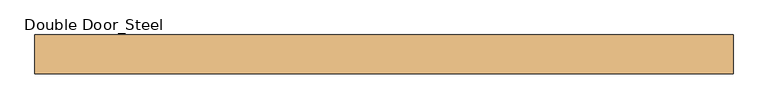
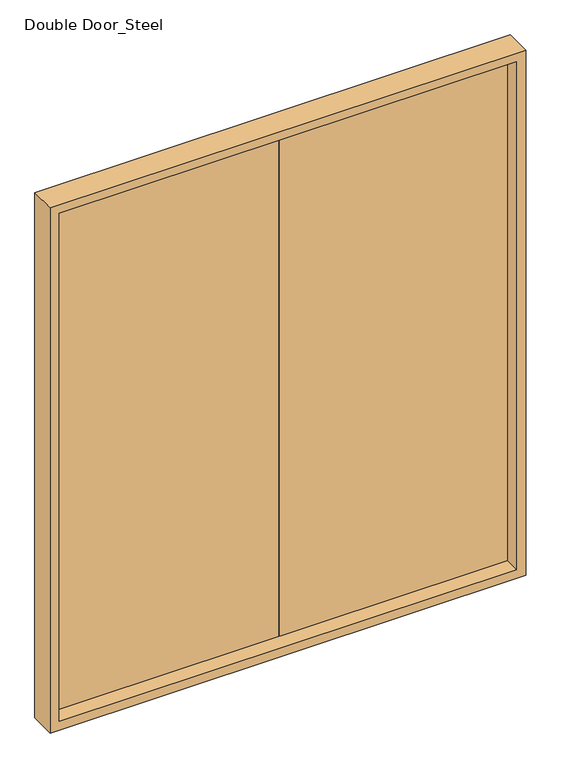
"""IFC4 building model written with IfcOpenShell, lengths in millimetres: door geometry, Double Door_Steel : H_DR_AR_B12_Double Door_Steel_W2000xH2100_0Hr."""

import ifcopenshell
import ifcopenshell.guid

model = None  # the IFC model being written
_history = None  # IfcOwnerHistory: only IFC2X3 demands one
_inside = {}  # id of a spatial element -> (the spatial element, [elements in it])
_under = {}  # id of a project, library or spatial element -> (it, [spatial elements below it])
_declared = {}  # id of a project -> (the project, [libraries it declares])
_typed = {}  # id of a type object -> (the type object, [elements of that type])
_made_of = {}  # id of a material, layer set ... -> (it, [elements and type objects made of it])


def new_model(schema):
    """Start an empty IFC model of exactly this schema.

    Asked for "IFC4X3", IfcOpenShell would pick the latest addendum, in which some entities
    have other attributes; the version numbers below select the first issue.
    IFC2X3 requires an IfcOwnerHistory on every rooted entity: one is made here for all.
    """
    global model, _history
    if schema == "IFC4X3":
        model = ifcopenshell.file(schema_version=(4, 3, 0, 0))
    else:
        model = ifcopenshell.file(schema=schema)
    _inside.clear()
    _under.clear()
    _declared.clear()
    _typed.clear()
    _made_of.clear()
    _history = None
    if model.schema == "IFC2X3":
        org = make("IfcOrganization", Name="unknown")
        user = make(
            "IfcPersonAndOrganization",
            ThePerson=make("IfcPerson", FamilyName="unknown"),
            TheOrganization=org,
        )
        app = make(
            "IfcApplication",
            ApplicationDeveloper=org,
            Version="unknown",
            ApplicationFullName="unknown",
            ApplicationIdentifier="unknown",
        )
        _history = make(
            "IfcOwnerHistory",
            OwningUser=user,
            OwningApplication=app,
            ChangeAction="ADDED",
            CreationDate=0,
        )
    return model


def make(cls, **values):
    """One entity of the class cls with the attributes given. An attribute that is None is left unset."""
    return model.create_entity(
        cls, **{name: value for name, value in values.items() if value is not None}
    )


def rooted(cls, **values):
    """An entity with a GlobalId (a new one), such as an element, a storey or a relation."""
    return make(cls, GlobalId=ifcopenshell.guid.new(), OwnerHistory=_history, **values)


def si_unit(unit_type, name, prefix=None):
    """IfcSIUnit, for example si_unit("LENGTHUNIT", "METRE", prefix="MILLI")."""
    return make("IfcSIUnit", UnitType=unit_type, Prefix=prefix, Name=name)


def assignment(units):
    """IfcUnitAssignment: the units of a project."""
    return None if units is None else make("IfcUnitAssignment", Units=units)


def point(xyz):
    """IfcCartesianPoint."""
    return None if xyz is None else make("IfcCartesianPoint", Coordinates=xyz)


def direction(xyz):
    """IfcDirection."""
    return None if xyz is None else make("IfcDirection", DirectionRatios=xyz)


def frame(location, z_axis=None, x_axis=None):
    """IfcAxis2Placement3D, a coordinate frame: its origin and axes. An axis left out is left unset."""
    return make(
        "IfcAxis2Placement3D",
        Location=point(location),
        Axis=direction(z_axis),
        RefDirection=direction(x_axis),
    )


def origin():
    """The frame at (0, 0, 0) with its axes left unset."""
    return frame((0.0, 0.0, 0.0))


def place(relative_to, where):
    """IfcLocalPlacement: puts the frame where relative to a parent placement (None: the world)."""
    return make(
        "IfcLocalPlacement", PlacementRelTo=relative_to, RelativePlacement=where
    )


def context(
    kind, dimensions, precision=None, world=None, true_north=None, identifier=None
):
    """IfcGeometricRepresentationContext, for example the 3D "Model" context."""
    return make(
        "IfcGeometricRepresentationContext",
        ContextIdentifier=identifier,
        ContextType=kind,
        CoordinateSpaceDimension=dimensions,
        Precision=precision,
        WorldCoordinateSystem=world,
        TrueNorth=true_north,
    )


def project(units=None, contexts=None):
    """IfcProject with its units and contexts."""
    return rooted(
        "IfcProject",
        Name="project",
        RepresentationContexts=contexts,
        UnitsInContext=assignment(units),
    )


def spatial(cls, under=None, at=None, **own):
    """A site, building, storey or space (cls), placed at a placement, below another one or the project."""
    s = rooted(cls, ObjectPlacement=at, **own)
    if under is not None:
        _under.setdefault(under.id(), (under, []))[1].append(s)
    return s


def polyline(points):
    """IfcPolyline through the points."""
    return make("IfcPolyline", Points=[point(p) for p in points])


def outline(outer, holes=None, kind="AREA"):
    """IfcArbitraryClosedProfileDef: a profile drawn as a closed curve; with holes, ...WithVoids."""
    if holes is None:
        return make("IfcArbitraryClosedProfileDef", ProfileType=kind, OuterCurve=outer)
    return make(
        "IfcArbitraryProfileDefWithVoids",
        ProfileType=kind,
        OuterCurve=outer,
        InnerCurves=holes,
    )


def extrude(swept, where, along, depth):
    """IfcExtrudedAreaSolid: the profile swept, set in the frame where, extruded along a direction by depth."""
    return make(
        "IfcExtrudedAreaSolid",
        SweptArea=swept,
        Position=where,
        ExtrudedDirection=direction(along),
        Depth=depth,
    )


def faces_of(points, faces, orient=None, outer=None):
    """IfcFace entities. A face is a list of loops; a loop is a list of indices into points, from 0.

    orient and outer hold one flag for each loop. By default every Orientation is true, the
    first loop of a face is its IfcFaceOuterBound and the others are IfcFaceBound.
    """
    made = []
    for i, loops in enumerate(faces):
        bounds = []
        for j, loop in enumerate(loops):
            is_outer = j == 0 if outer is None else outer[i][j]
            bounds.append(
                make(
                    "IfcFaceOuterBound" if is_outer else "IfcFaceBound",
                    Bound=make("IfcPolyLoop", Polygon=[points[k] for k in loop]),
                    Orientation=True if orient is None else orient[i][j],
                )
            )
        made.append(make("IfcFace", Bounds=bounds))
    return made


def faceted_brep(points, faces, orient=None, outer=None, voids=None):
    """IfcFacetedBrep: a solid bounded by flat faces; with voids (closed shells), ...WithVoids."""
    shared = [point(p) for p in points]
    hull = make("IfcClosedShell", CfsFaces=faces_of(shared, faces, orient, outer))
    if voids is None:
        return make("IfcFacetedBrep", Outer=hull)
    return make(
        "IfcFacetedBrepWithVoids",
        Outer=hull,
        Voids=[
            make(cls, CfsFaces=faces_of(shared, fs, o, b)) for cls, fs, o, b in voids
        ],
    )


def shape(context_of_items, identifier, shape_type, items):
    """IfcShapeRepresentation: the items that make up one representation, for example the "Body"."""
    return make(
        "IfcShapeRepresentation",
        ContextOfItems=context_of_items,
        RepresentationIdentifier=identifier,
        RepresentationType=shape_type,
        Items=items,
    )


def source(mapping_origin, context_of_items, identifier, shape_type, items):
    """IfcRepresentationMap: a shape defined once, which mapped items show again and again."""
    return make(
        "IfcRepresentationMap",
        MappingOrigin=mapping_origin,
        MappedRepresentation=shape(context_of_items, identifier, shape_type, items),
    )


def transform(
    local_origin,
    x_axis=None,
    y_axis=None,
    z_axis=None,
    scale=None,
    scale2=None,
    scale3=None,
    uniform=True,
):
    """IfcCartesianTransformationOperator3D, or its non-uniform kind. x_axis, y_axis, z_axis: its Axis1, 2, 3."""
    if uniform:
        return make(
            "IfcCartesianTransformationOperator3D",
            Axis1=direction(x_axis),
            Axis2=direction(y_axis),
            LocalOrigin=point(local_origin),
            Scale=scale,
            Axis3=direction(z_axis),
        )
    return make(
        "IfcCartesianTransformationOperator3DnonUniform",
        Axis1=direction(x_axis),
        Axis2=direction(y_axis),
        LocalOrigin=point(local_origin),
        Scale=scale,
        Axis3=direction(z_axis),
        Scale2=scale2,
        Scale3=scale3,
    )


def mapped(mapping_source, mapping_target):
    """IfcMappedItem: shows the shape of a source again, moved by a transform."""
    return make(
        "IfcMappedItem", MappingSource=mapping_source, MappingTarget=mapping_target
    )


def made_of(thing, what):
    """Note that an element or type object is made of a material, layer set ...; save() writes the relation."""
    if what is not None:
        _made_of.setdefault(what.id(), (what, []))[1].append(thing)
    return thing


def element(
    cls,
    number,
    at=None,
    inside=None,
    cuts=None,
    type_object=None,
    material=None,
    context=None,
    identifier="Body",
    shape_type=None,
    held_by="IfcProductDefinitionShape",
    body=None,
    shapes=None,
    **own,
):
    """One element of the class cls, such as IfcWall. Its Tag is "e" and its number.

    at: its placement. inside: the storey or other place that contains it. cuts: it is an
    opening in that element (IfcRelVoidsElement). A single representation is given by context,
    identifier, shape_type and body (its items); several are given by shapes. held_by: the class
    of the entity that holds the representations. save() writes the other relations.
    """
    e = rooted(cls, Tag="e%d" % number, ObjectPlacement=at, **own)
    if body is not None:
        shapes = [shape(context, identifier, shape_type, body)]
    if shapes is not None:
        e.Representation = make(held_by, Representations=shapes)
    if inside is not None:
        _inside.setdefault(inside.id(), (inside, []))[1].append(e)
    if cuts is not None:
        rooted(
            "IfcRelVoidsElement", RelatingBuildingElement=cuts, RelatedOpeningElement=e
        )
    if type_object is not None:
        _typed.setdefault(type_object.id(), (type_object, []))[1].append(e)
    return made_of(e, material)


def aggregate(whole, parts):
    """IfcRelAggregates: a whole, such as a stair, and the parts it consists of."""
    return rooted("IfcRelAggregates", RelatingObject=whole, RelatedObjects=parts)


def save(model, path):
    """Write the relations noted so far, then the file.

    IfcRelAggregates (storeys below a building ...), IfcRelContainedInSpatialStructure (elements
    in a storey), IfcRelDefinesByType, IfcRelAssociatesMaterial and IfcRelDeclares: one each for
    every whole, place, type object, material and project.
    """
    for whole, parts in _under.values():
        aggregate(whole, parts)
    for where, things in _inside.values():
        rooted(
            "IfcRelContainedInSpatialStructure",
            RelatedElements=things,
            RelatingStructure=where,
        )
    for kind, things in _typed.values():
        rooted("IfcRelDefinesByType", RelatedObjects=things, RelatingType=kind)
    for what, things in _made_of.values():
        rooted("IfcRelAssociatesMaterial", RelatedObjects=things, RelatingMaterial=what)
    for by, libraries in _declared.values():
        rooted("IfcRelDeclares", RelatingContext=by, RelatedDefinitions=libraries)
    model.write(path)


def double_door_steel_00e42113(model_context):
    return source(origin(), model_context, "Body", "SolidModel", [
        extrude(outline(polyline([(880.0, 10.0), (0.0, 10.0), (0.0, 50.0), (880.0, 50.0), (880.0, 10.0)])), frame((0.0, 0.0, 20.0), z_axis=(0.0, 0.0, 1.0), x_axis=(1.0, 0.0, 0.0)), (0.0, 0.0, 1.0), 2060.0),
        extrude(outline(polyline([(0.0, 10.0), (-880.0, 10.0), (-880.0, 50.0), (0.0, 50.0), (0.0, 10.0)])), frame((0.0, 0.0, 20.0), z_axis=(0.0, 0.0, 1.0), x_axis=(1.0, 0.0, 0.0)), (0.0, 0.0, 1.0), 2060.0),
        faceted_brep([(900.0, -50.0, 2100.0), (900.0, 50.0, 2100.0), (-900.0, 50.0, 2100.0), (-900.0, -50.0, 2100.0), (865.0, 10.0, 2065.0), (865.0, -50.0, 2065.0), (-865.0, -50.0, 2065.0), (-865.0, 10.0, 2065.0), (880.0, 50.0, 2080.0), (880.0, 10.0, 2080.0), (-880.0, 10.0, 2080.0), (-880.0, 50.0, 2080.0), (-900.0, 50.0, 0.0), (-900.0, -50.0, 0.0), (-865.0, -50.0, 35.0), (-865.0, 10.0, 35.0), (-880.0, 10.0, 20.0), (-880.0, 50.0, 20.0), (900.0, 50.0, 0.0), (880.0, 50.0, 20.0), (900.0, -50.0, 0.0), (865.0, -50.0, 35.0), (865.0, 10.0, 35.0), (880.0, 10.0, 20.0)], [[[0, 1, 2, 3]], [[4, 5, 6, 7]], [[8, 9, 10, 11]], [[3, 2, 12, 13]], [[7, 6, 14, 15]], [[11, 10, 16, 17]], [[18, 12, 2, 1], [8, 11, 17, 19]], [[13, 12, 18, 20]], [[0, 3, 13, 20], [21, 14, 6, 5]], [[15, 14, 21, 22]], [[23, 16, 10, 9], [4, 7, 15, 22]], [[17, 16, 23, 19]], [[20, 18, 1, 0]], [[22, 21, 5, 4]], [[19, 23, 9, 8]]]),
    ])


if __name__ == "__main__":
    model = new_model("IFC4")
    model_context = context("Model", 3, world=origin())
    ifc_project = project(units=[si_unit("LENGTHUNIT", "METRE", prefix="MILLI")], contexts=[model_context])
    site = spatial("IfcSite", under=ifc_project)
    building = spatial("IfcBuilding", under=site)
    placement = place(None, origin())
    double_door_steel_shape = double_door_steel_00e42113(model_context)
    element("IfcDoor", 1, ObjectType="Double Door_Steel : H_DR_AR_B12_Double Door_Steel_W2000xH2100_0Hr", at=placement, inside=building, context=model_context, shape_type="MappedRepresentation", body=[
        mapped(double_door_steel_shape, transform((0.0, 0.0, 0.0), x_axis=(1.0, 0.0, 0.0), y_axis=(0.0, 1.0, 0.0), z_axis=(0.0, 0.0, 1.0))),
    ])
    save(model, "model.ifc")

# Revit data of these elements
# Type "Double Door_Steel : H_DR_AR_B12_Double Door_Steel_W2000xH2100_0Hr"
#   Type Mark = "SD2"
#   프레임 = ""
#   철물 = ""
#   유리/마감 = ""
#   위치/개소 = ""
#   부호 = "1/SD"
#   문번호 = ""
#   문기호 = "SD"
#   Analytic Construction = "<None>"
#   Height = 2100 mm
#   Width = 1800 mm
#   Define Thermal Properties by = 1
#   문 틀 = none
#   문 = none
#   Function = (empty or 0)
#   Assembly Code = ""
#   Wall Closure = (empty or 0)
